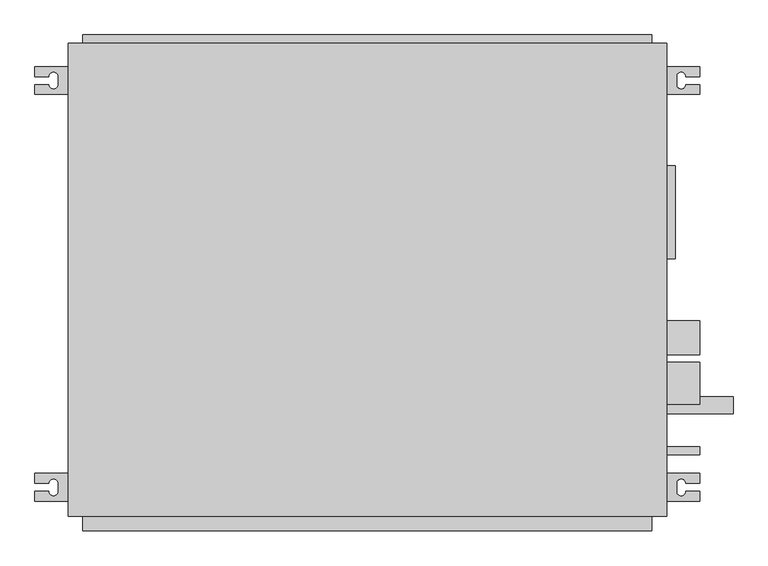
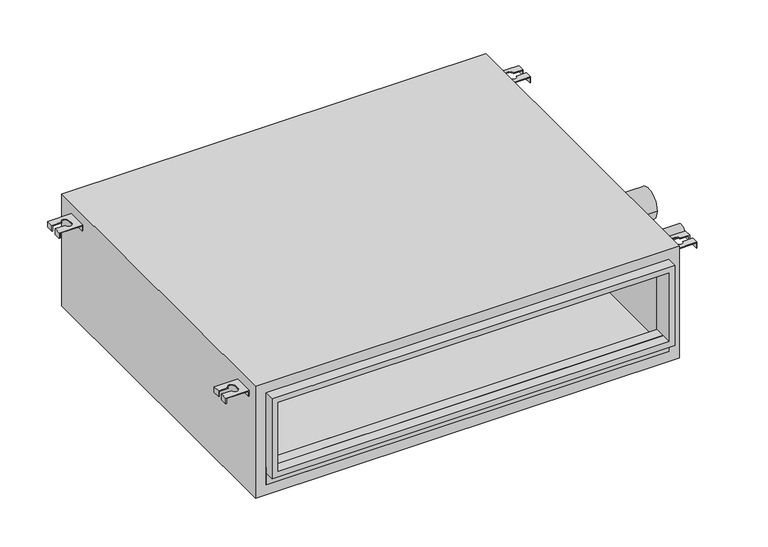
"""IFC4 building model written with IfcOpenShell, lengths in millimetres: proxy geometry, PEFY-P-NMAU-E_Medium_Static_Ducted : PEFY-P18NMAU-E."""

import ifcopenshell
import ifcopenshell.guid

model = None  # the IFC model being written
_history = None  # IfcOwnerHistory: only IFC2X3 demands one
_inside = {}  # id of a spatial element -> (the spatial element, [elements in it])
_under = {}  # id of a project, library or spatial element -> (it, [spatial elements below it])
_declared = {}  # id of a project -> (the project, [libraries it declares])
_typed = {}  # id of a type object -> (the type object, [elements of that type])
_made_of = {}  # id of a material, layer set ... -> (it, [elements and type objects made of it])


def new_model(schema):
    """Start an empty IFC model of exactly this schema.

    Asked for "IFC4X3", IfcOpenShell would pick the latest addendum, in which some entities
    have other attributes; the version numbers below select the first issue.
    IFC2X3 requires an IfcOwnerHistory on every rooted entity: one is made here for all.
    """
    global model, _history
    if schema == "IFC4X3":
        model = ifcopenshell.file(schema_version=(4, 3, 0, 0))
    else:
        model = ifcopenshell.file(schema=schema)
    _inside.clear()
    _under.clear()
    _declared.clear()
    _typed.clear()
    _made_of.clear()
    _history = None
    if model.schema == "IFC2X3":
        org = make("IfcOrganization", Name="unknown")
        user = make(
            "IfcPersonAndOrganization",
            ThePerson=make("IfcPerson", FamilyName="unknown"),
            TheOrganization=org,
        )
        app = make(
            "IfcApplication",
            ApplicationDeveloper=org,
            Version="unknown",
            ApplicationFullName="unknown",
            ApplicationIdentifier="unknown",
        )
        _history = make(
            "IfcOwnerHistory",
            OwningUser=user,
            OwningApplication=app,
            ChangeAction="ADDED",
            CreationDate=0,
        )
    return model


def make(cls, **values):
    """One entity of the class cls with the attributes given. An attribute that is None is left unset."""
    return model.create_entity(
        cls, **{name: value for name, value in values.items() if value is not None}
    )


def rooted(cls, **values):
    """An entity with a GlobalId (a new one), such as an element, a storey or a relation."""
    return make(cls, GlobalId=ifcopenshell.guid.new(), OwnerHistory=_history, **values)


def si_unit(unit_type, name, prefix=None):
    """IfcSIUnit, for example si_unit("LENGTHUNIT", "METRE", prefix="MILLI")."""
    return make("IfcSIUnit", UnitType=unit_type, Prefix=prefix, Name=name)


def assignment(units):
    """IfcUnitAssignment: the units of a project."""
    return None if units is None else make("IfcUnitAssignment", Units=units)


def point(xyz):
    """IfcCartesianPoint."""
    return None if xyz is None else make("IfcCartesianPoint", Coordinates=xyz)


def direction(xyz):
    """IfcDirection."""
    return None if xyz is None else make("IfcDirection", DirectionRatios=xyz)


def frame(location, z_axis=None, x_axis=None):
    """IfcAxis2Placement3D, a coordinate frame: its origin and axes. An axis left out is left unset."""
    return make(
        "IfcAxis2Placement3D",
        Location=point(location),
        Axis=direction(z_axis),
        RefDirection=direction(x_axis),
    )


def frame_2d(location, x_axis=None):
    """IfcAxis2Placement2D, a coordinate frame in the plane: its origin and x axis."""
    return make(
        "IfcAxis2Placement2D", Location=point(location), RefDirection=direction(x_axis)
    )


def origin():
    """The frame at (0, 0, 0) with its axes left unset."""
    return frame((0.0, 0.0, 0.0))


def place(relative_to, where):
    """IfcLocalPlacement: puts the frame where relative to a parent placement (None: the world)."""
    return make(
        "IfcLocalPlacement", PlacementRelTo=relative_to, RelativePlacement=where
    )


def context(
    kind, dimensions, precision=None, world=None, true_north=None, identifier=None
):
    """IfcGeometricRepresentationContext, for example the 3D "Model" context."""
    return make(
        "IfcGeometricRepresentationContext",
        ContextIdentifier=identifier,
        ContextType=kind,
        CoordinateSpaceDimension=dimensions,
        Precision=precision,
        WorldCoordinateSystem=world,
        TrueNorth=true_north,
    )


def project(units=None, contexts=None):
    """IfcProject with its units and contexts."""
    return rooted(
        "IfcProject",
        Name="project",
        RepresentationContexts=contexts,
        UnitsInContext=assignment(units),
    )


def spatial(cls, under=None, at=None, **own):
    """A site, building, storey or space (cls), placed at a placement, below another one or the project."""
    s = rooted(cls, ObjectPlacement=at, **own)
    if under is not None:
        _under.setdefault(under.id(), (under, []))[1].append(s)
    return s


def polyline(points):
    """IfcPolyline through the points."""
    return make("IfcPolyline", Points=[point(p) for p in points])


def circle_curve(where, radius):
    """IfcCircle in the frame where."""
    return make("IfcCircle", Position=where, Radius=radius)


def trimmed(basis, trim1, trim2, sense, master):
    """IfcTrimmedCurve: the piece of a basis curve between two trims."""
    return make(
        "IfcTrimmedCurve",
        BasisCurve=basis,
        Trim1=trim1,
        Trim2=trim2,
        SenseAgreement=sense,
        MasterRepresentation=master,
    )


def segment(curve, same_sense, transition):
    """IfcCompositeCurveSegment."""
    return make(
        "IfcCompositeCurveSegment",
        Transition=transition,
        SameSense=same_sense,
        ParentCurve=curve,
    )


def composite_curve(segments, self_intersect=None):
    """IfcCompositeCurve: segments joined end to end."""
    return make("IfcCompositeCurve", Segments=segments, SelfIntersect=self_intersect)


def outline(outer, holes=None, kind="AREA"):
    """IfcArbitraryClosedProfileDef: a profile drawn as a closed curve; with holes, ...WithVoids."""
    if holes is None:
        return make("IfcArbitraryClosedProfileDef", ProfileType=kind, OuterCurve=outer)
    return make(
        "IfcArbitraryProfileDefWithVoids",
        ProfileType=kind,
        OuterCurve=outer,
        InnerCurves=holes,
    )


def extrude(swept, where, along, depth):
    """IfcExtrudedAreaSolid: the profile swept, set in the frame where, extruded along a direction by depth."""
    return make(
        "IfcExtrudedAreaSolid",
        SweptArea=swept,
        Position=where,
        ExtrudedDirection=direction(along),
        Depth=depth,
    )


def shape(context_of_items, identifier, shape_type, items):
    """IfcShapeRepresentation: the items that make up one representation, for example the "Body"."""
    return make(
        "IfcShapeRepresentation",
        ContextOfItems=context_of_items,
        RepresentationIdentifier=identifier,
        RepresentationType=shape_type,
        Items=items,
    )


def source(mapping_origin, context_of_items, identifier, shape_type, items):
    """IfcRepresentationMap: a shape defined once, which mapped items show again and again."""
    return make(
        "IfcRepresentationMap",
        MappingOrigin=mapping_origin,
        MappedRepresentation=shape(context_of_items, identifier, shape_type, items),
    )


def transform(
    local_origin,
    x_axis=None,
    y_axis=None,
    z_axis=None,
    scale=None,
    scale2=None,
    scale3=None,
    uniform=True,
):
    """IfcCartesianTransformationOperator3D, or its non-uniform kind. x_axis, y_axis, z_axis: its Axis1, 2, 3."""
    if uniform:
        return make(
            "IfcCartesianTransformationOperator3D",
            Axis1=direction(x_axis),
            Axis2=direction(y_axis),
            LocalOrigin=point(local_origin),
            Scale=scale,
            Axis3=direction(z_axis),
        )
    return make(
        "IfcCartesianTransformationOperator3DnonUniform",
        Axis1=direction(x_axis),
        Axis2=direction(y_axis),
        LocalOrigin=point(local_origin),
        Scale=scale,
        Axis3=direction(z_axis),
        Scale2=scale2,
        Scale3=scale3,
    )


def mapped(mapping_source, mapping_target):
    """IfcMappedItem: shows the shape of a source again, moved by a transform."""
    return make(
        "IfcMappedItem", MappingSource=mapping_source, MappingTarget=mapping_target
    )


def made_of(thing, what):
    """Note that an element or type object is made of a material, layer set ...; save() writes the relation."""
    if what is not None:
        _made_of.setdefault(what.id(), (what, []))[1].append(thing)
    return thing


def element(
    cls,
    number,
    at=None,
    inside=None,
    cuts=None,
    type_object=None,
    material=None,
    context=None,
    identifier="Body",
    shape_type=None,
    held_by="IfcProductDefinitionShape",
    body=None,
    shapes=None,
    **own,
):
    """One element of the class cls, such as IfcWall. Its Tag is "e" and its number.

    at: its placement. inside: the storey or other place that contains it. cuts: it is an
    opening in that element (IfcRelVoidsElement). A single representation is given by context,
    identifier, shape_type and body (its items); several are given by shapes. held_by: the class
    of the entity that holds the representations. save() writes the other relations.
    """
    e = rooted(cls, Tag="e%d" % number, ObjectPlacement=at, **own)
    if body is not None:
        shapes = [shape(context, identifier, shape_type, body)]
    if shapes is not None:
        e.Representation = make(held_by, Representations=shapes)
    if inside is not None:
        _inside.setdefault(inside.id(), (inside, []))[1].append(e)
    if cuts is not None:
        rooted(
            "IfcRelVoidsElement", RelatingBuildingElement=cuts, RelatedOpeningElement=e
        )
    if type_object is not None:
        _typed.setdefault(type_object.id(), (type_object, []))[1].append(e)
    return made_of(e, material)


def aggregate(whole, parts):
    """IfcRelAggregates: a whole, such as a stair, and the parts it consists of."""
    return rooted("IfcRelAggregates", RelatingObject=whole, RelatedObjects=parts)


def save(model, path):
    """Write the relations noted so far, then the file.

    IfcRelAggregates (storeys below a building ...), IfcRelContainedInSpatialStructure (elements
    in a storey), IfcRelDefinesByType, IfcRelAssociatesMaterial and IfcRelDeclares: one each for
    every whole, place, type object, material and project.
    """
    for whole, parts in _under.values():
        aggregate(whole, parts)
    for where, things in _inside.values():
        rooted(
            "IfcRelContainedInSpatialStructure",
            RelatedElements=things,
            RelatingStructure=where,
        )
    for kind, things in _typed.values():
        rooted("IfcRelDefinesByType", RelatedObjects=things, RelatingType=kind)
    for what, things in _made_of.values():
        rooted("IfcRelAssociatesMaterial", RelatedObjects=things, RelatingMaterial=what)
    for by, libraries in _declared.values():
        rooted("IfcRelDeclares", RelatingContext=by, RelatedDefinitions=libraries)
    model.write(path)


def plane_surface(at):
    """IfcPlane: the flat surface through the origin of the frame at, square to its z axis."""
    return make("IfcPlane", Position=at)


def revolved_surface(curve, axis_point, axis_direction):
    """IfcSurfaceOfRevolution: the curve turned about the line through axis_point along axis_direction."""
    return make(
        "IfcSurfaceOfRevolution",
        SweptCurve=make("IfcArbitraryOpenProfileDef", ProfileType="CURVE", Curve=curve),
        AxisPosition=make("IfcAxis1Placement", Location=point(axis_point), Axis=direction(axis_direction)),
    )


def advanced_brep(points, edges, surfaces, faces):
    """IfcAdvancedBrep: a solid bounded by faces that lie on surfaces and meet in shared edges.

    An edge is (start, end): straight between two places in points (the first is 0);
    or (start, end, curve); or (start, end, curve, False) where it runs against its curve.
    A face is (place in surfaces, loops), or (place, loops, False) where it looks against
    its surface's normal. A loop lists edges by number (the first is 1), with a minus sign
    where the edge is run from its end to its start. The first loop is the outer one.
    """
    corners = [point(p) for p in points]
    vertices = [make("IfcVertexPoint", VertexGeometry=c) for c in corners]
    made = []
    for start, end, *more in edges:
        made.append(
            make(
                "IfcEdgeCurve",
                EdgeStart=vertices[start],
                EdgeEnd=vertices[end],
                EdgeGeometry=more[0] if more else make("IfcPolyline", Points=[corners[start], corners[end]]),
                SameSense=more[1] if len(more) > 1 else True,
            )
        )
    hull = []
    for where, loops, *sense in faces:
        bounds = []
        for j, loop in enumerate(loops):
            ring = [make("IfcOrientedEdge", EdgeElement=made[abs(k) - 1], Orientation=k > 0) for k in loop]
            bounds.append(
                make(
                    "IfcFaceOuterBound" if j == 0 else "IfcFaceBound",
                    Bound=make("IfcEdgeLoop", EdgeList=ring),
                    Orientation=True,
                )
            )
        hull.append(make("IfcAdvancedFace", Bounds=bounds, FaceSurface=surfaces[where], SameSense=sense[0] if sense else True))
    return make("IfcAdvancedBrep", Outer=make("IfcClosedShell", CfsFaces=hull))


def mechanical_equipment_7e022f85(model_context):
    return source(origin(), model_context, "Body", "SolidModel", [
        advanced_brep(
        [(-510.074743, -231.05, 249.2375), (-510.074743, -246.05, 249.2375), (-489.068493, -246.05, 249.2375), (-475.068493, -246.05, 249.2375), (-475.068493, -258.05, 249.2375), (-489.068493, -258.05, 249.2375), (-510.074743, -258.05, 249.2375), (-510.074743, -273.05, 249.2375), (-460.068493, -273.05, 249.2375), (-460.068493, -231.05, 249.2375), (-510.074743, -231.05, 236.4972162), (-508.486743, -231.05, 236.4972162), (-508.486743, -246.05, 236.4972162), (-510.074743, -246.05, 236.4972162), (-508.486743, -273.05, 236.4972162), (-510.074743, -273.05, 236.4972162), (-510.074743, -258.05, 236.4972162), (-508.486743, -258.05, 236.4972162), (-460.068493, -231.05, 236.4972162), (-460.068493, -273.05, 236.4972162), (-461.656493, -273.05, 236.4972162), (-461.656493, -231.05, 236.4972162), (-508.486743, -246.05, 247.65), (-489.068493, -246.05, 247.65), (-508.486743, -231.05, 247.65), (-461.656493, -231.05, 247.65), (-508.486743, -258.05, 247.65), (-508.486743, -273.05, 247.65), (-489.068493, -258.05, 247.65), (-461.656493, -273.05, 247.65), (-475.068493, -258.05, 247.65), (-475.068493, -246.05, 247.65)],
        [
            (0, 1),
            (1, 2),
            (2, 3, circle_curve(frame((-482.068493, -246.05, 249.2375), z_axis=(0.0, 0.0, -1.0), x_axis=(1.0, 0.0, 0.0)), 7.0)),
            (3, 4),
            (4, 5, circle_curve(frame((-482.068493, -258.05, 249.2375), z_axis=(0.0, 0.0, -1.0), x_axis=(1.0, 0.0, 0.0)), 7.0)),
            (5, 6),
            (6, 7),
            (7, 8),
            (8, 9),
            (9, 0),
            (10, 11),
            (11, 12),
            (12, 13),
            (13, 10),
            (14, 15),
            (15, 16),
            (16, 17),
            (17, 14),
            (18, 19),
            (19, 20),
            (20, 21),
            (21, 18),
            (13, 1),
            (0, 10),
            (12, 22),
            (22, 23),
            (23, 2),
            (11, 24),
            (24, 22),
            (9, 18),
            (21, 25),
            (25, 24),
            (17, 26),
            (26, 27),
            (27, 14),
            (5, 28),
            (28, 26),
            (16, 6),
            (15, 7),
            (27, 29),
            (29, 20),
            (19, 8),
            (29, 25),
            (30, 31),
            (31, 23, circle_curve(frame((-482.068493, -246.05, 247.65), z_axis=(0.0, 0.0, 1.0), x_axis=(1.0, 0.0, 0.0)), 7.0)),
            (28, 30, circle_curve(frame((-482.068493, -258.05, 247.65), z_axis=(0.0, 0.0, 1.0), x_axis=(1.0, 0.0, 0.0)), 7.0)),
            (4, 30),
            (31, 3),
        ],
        [
            plane_surface(frame((-510.074743, -231.05, 249.2375), z_axis=(0.0, 0.0, 1.0), x_axis=(0.0, -1.0, 0.0))),
            plane_surface(frame((-510.074743, -231.05, 236.4972162), z_axis=(0.0, 0.0, -1.0), x_axis=(0.0, 1.0, 0.0))),
            plane_surface(frame((-510.074743, -231.05, 249.2375), z_axis=(-1.0, 0.0, 0.0), x_axis=(0.0, 0.0, -1.0))),
            plane_surface(frame((-510.074743, -246.05, 249.2375), z_axis=(0.0, -1.0, 0.0), x_axis=(0.0, 0.0, -1.0))),
            plane_surface(frame((-508.486743, -246.05, 249.2375), z_axis=(1.0, 0.0, 0.0), x_axis=(0.0, 0.0, -1.0))),
            plane_surface(frame((-508.486743, -231.05, 249.2375), z_axis=(0.0, 1.0, 0.0), x_axis=(0.0, 0.0, -1.0))),
            plane_surface(frame((-508.486743, -273.05, 249.2375), z_axis=(1.0, 0.0, 0.0), x_axis=(0.0, 0.0, -1.0))),
            plane_surface(frame((-508.486743, -258.05, 249.2375), z_axis=(0.0, 1.0, 0.0), x_axis=(0.0, 0.0, -1.0))),
            plane_surface(frame((-510.074743, -258.05, 249.2375), z_axis=(-1.0, 0.0, 0.0), x_axis=(0.0, 0.0, -1.0))),
            plane_surface(frame((-510.074743, -273.05, 249.2375), z_axis=(0.0, -1.0, 0.0), x_axis=(0.0, 0.0, -1.0))),
            plane_surface(frame((-461.656493, -231.05, 249.2375), z_axis=(-1.0, 0.0, 0.0), x_axis=(0.0, 0.0, -1.0))),
            plane_surface(frame((-460.068493, -273.05, 249.2375), z_axis=(1.0, 0.0, 0.0), x_axis=(0.0, 0.0, -1.0))),
            plane_surface(frame((-475.068493, -258.05, 247.65), z_axis=(0.0, 0.0, -1.0), x_axis=(0.0, 1.0, 0.0))),
            revolved_surface(polyline([(-475.068493, -258.05, 247.65), (-475.068493, -258.05, 249.2375)]), (-482.068493, -258.05, 247.65), (0.0, 0.0, -1.0)),
            revolved_surface(polyline([(-475.068493, -246.05, 247.65), (-475.068493, -246.05, 249.2375)]), (-482.068493, -246.05, 247.65), (0.0, 0.0, -1.0)),
            plane_surface(frame((-475.068493, -246.05, 249.2375), z_axis=(-1.0, 0.0, 0.0), x_axis=(0.0, 0.0, -1.0))),
        ],
        [
            (0, [[1, 2, 3, 4, 5, 6, 7, 8, 9, 10]]),
            (1, [[11, 12, 13, 14]]),
            (1, [[15, 16, 17, 18]]),
            (1, [[19, 20, 21, 22]]),
            (2, [[23, -1, 24, -14]]),
            (3, [[-2, -23, -13, 25, 26, 27]]),
            (4, [[-12, 28, 29, -25]]),
            (5, [[-10, 30, -22, 31, 32, -28, -11, -24]]),
            (6, [[-18, 33, 34, 35]]),
            (7, [[-6, 36, 37, -33, -17, 38]]),
            (8, [[39, -7, -38, -16]]),
            (9, [[-8, -39, -15, -35, 40, 41, -20, 42]]),
            (10, [[-21, -41, 43, -31]]),
            (11, [[-30, -9, -42, -19]]),
            (12, [[44, 45, -26, -29, -32, -43, -40, -34, -37, 46]]),
            (13, [[-5, 47, -46, -36]]),
            (14, [[-3, -27, -45, 48]]),
            (15, [[-4, -48, -44, -47]]),
        ],
    ),
        advanced_brep(
        [(490.050257, -231.05, 249.2375), (440.044007, -231.05, 249.2375), (440.044007, -273.05, 249.2375), (490.050257, -273.05, 249.2375), (490.050257, -258.05, 249.2375), (469.044007, -258.05, 249.2375), (455.044007, -258.05, 249.2375), (455.044007, -246.05, 249.2375), (469.044007, -246.05, 249.2375), (490.050257, -246.05, 249.2375), (490.050257, -231.05, 236.4972162), (490.050257, -246.05, 236.4972162), (488.462257, -246.05, 236.4972162), (488.462257, -231.05, 236.4972162), (488.462257, -273.05, 236.4972162), (488.462257, -258.05, 236.4972162), (490.050257, -258.05, 236.4972162), (490.050257, -273.05, 236.4972162), (440.044007, -231.05, 236.4972162), (441.632007, -231.05, 236.4972162), (441.632007, -273.05, 236.4972162), (440.044007, -273.05, 236.4972162), (469.044007, -246.05, 247.65), (488.462257, -246.05, 247.65), (488.462257, -231.05, 247.65), (441.632007, -231.05, 247.65), (488.462257, -273.05, 247.65), (488.462257, -258.05, 247.65), (469.044007, -258.05, 247.65), (441.632007, -273.05, 247.65), (455.044007, -258.05, 247.65), (455.044007, -246.05, 247.65)],
        [
            (0, 1),
            (1, 2),
            (2, 3),
            (3, 4),
            (4, 5),
            (5, 6, circle_curve(frame((462.044007, -258.05, 249.2375), z_axis=(0.0, 0.0, -1.0), x_axis=(-1.0, 0.0, 0.0)), 7.0)),
            (6, 7),
            (7, 8, circle_curve(frame((462.044007, -246.05, 249.2375), z_axis=(0.0, 0.0, -1.0), x_axis=(-1.0, 0.0, 0.0)), 7.0)),
            (8, 9),
            (9, 0),
            (10, 11),
            (11, 12),
            (12, 13),
            (13, 10),
            (14, 15),
            (15, 16),
            (16, 17),
            (17, 14),
            (18, 19),
            (19, 20),
            (20, 21),
            (21, 18),
            (10, 0),
            (9, 11),
            (8, 22),
            (22, 23),
            (23, 12),
            (23, 24),
            (24, 13),
            (24, 25),
            (25, 19),
            (18, 1),
            (14, 26),
            (26, 27),
            (27, 15),
            (4, 16),
            (27, 28),
            (28, 5),
            (3, 17),
            (2, 21),
            (20, 29),
            (29, 26),
            (25, 29),
            (30, 28, circle_curve(frame((462.044007, -258.05, 247.65), z_axis=(0.0, 0.0, 1.0), x_axis=(-1.0, 0.0, 0.0)), 7.0)),
            (22, 31, circle_curve(frame((462.044007, -246.05, 247.65), z_axis=(0.0, 0.0, 1.0), x_axis=(-1.0, 0.0, 0.0)), 7.0)),
            (31, 30),
            (30, 6),
            (7, 31),
        ],
        [
            plane_surface(frame((490.050257, -231.05, 249.2375), z_axis=(0.0, 0.0, 1.0), x_axis=(0.0, -1.0, 0.0))),
            plane_surface(frame((490.050257, -231.05, 236.4972162), z_axis=(0.0, 0.0, -1.0), x_axis=(0.0, 1.0, 0.0))),
            plane_surface(frame((490.050257, -231.05, 249.2375), z_axis=(1.0, 0.0, 0.0), x_axis=(0.0, 0.0, -1.0))),
            plane_surface(frame((490.050257, -246.05, 249.2375), z_axis=(0.0, -1.0, 0.0), x_axis=(0.0, 0.0, -1.0))),
            plane_surface(frame((488.462257, -246.05, 249.2375), z_axis=(-1.0, 0.0, 0.0), x_axis=(0.0, 0.0, -1.0))),
            plane_surface(frame((488.462257, -231.05, 249.2375), z_axis=(0.0, 1.0, 0.0), x_axis=(0.0, 0.0, -1.0))),
            plane_surface(frame((488.462257, -273.05, 249.2375), z_axis=(-1.0, 0.0, 0.0), x_axis=(0.0, 0.0, -1.0))),
            plane_surface(frame((488.462257, -258.05, 249.2375), z_axis=(0.0, 1.0, 0.0), x_axis=(0.0, 0.0, -1.0))),
            plane_surface(frame((490.050257, -258.05, 249.2375), z_axis=(1.0, 0.0, 0.0), x_axis=(0.0, 0.0, -1.0))),
            plane_surface(frame((490.050257, -273.05, 249.2375), z_axis=(0.0, -1.0, 0.0), x_axis=(0.0, 0.0, -1.0))),
            plane_surface(frame((441.632007, -231.05, 249.2375), z_axis=(1.0, 0.0, 0.0), x_axis=(0.0, 0.0, -1.0))),
            plane_surface(frame((440.044007, -273.05, 249.2375), z_axis=(-1.0, 0.0, 0.0), x_axis=(0.0, 0.0, -1.0))),
            plane_surface(frame((455.044007, -258.05, 247.65), z_axis=(0.0, 0.0, -1.0), x_axis=(0.0, 1.0, 0.0))),
            revolved_surface(polyline([(455.044007, -258.05, 247.65), (455.044007, -258.05, 249.2375)]), (462.044007, -258.05, 247.65), (0.0, 0.0, -1.0)),
            revolved_surface(polyline([(455.044007, -246.05, 247.65), (455.044007, -246.05, 249.2375)]), (462.044007, -246.05, 247.65), (0.0, 0.0, -1.0)),
            plane_surface(frame((455.044007, -246.05, 249.2375), z_axis=(1.0, 0.0, 0.0), x_axis=(0.0, 0.0, -1.0))),
        ],
        [
            (0, [[1, 2, 3, 4, 5, 6, 7, 8, 9, 10]]),
            (1, [[11, 12, 13, 14]]),
            (1, [[15, 16, 17, 18]]),
            (1, [[19, 20, 21, 22]]),
            (2, [[-11, 23, -10, 24]]),
            (3, [[25, 26, 27, -12, -24, -9]]),
            (4, [[-27, 28, 29, -13]]),
            (5, [[-23, -14, -29, 30, 31, -19, 32, -1]]),
            (6, [[33, 34, 35, -15]]),
            (7, [[36, -16, -35, 37, 38, -5]]),
            (8, [[-17, -36, -4, 39]]),
            (9, [[40, -21, 41, 42, -33, -18, -39, -3]]),
            (10, [[-31, 43, -41, -20]]),
            (11, [[-22, -40, -2, -32]]),
            (12, [[44, -37, -34, -42, -43, -30, -28, -26, 45, 46]]),
            (13, [[-38, -44, 47, -6]]),
            (14, [[48, -45, -25, -8]]),
            (15, [[-47, -46, -48, -7]]),
        ],
    ),
        advanced_brep(
        [(-510.074743, 339.0, 249.2375), (-460.068493, 339.0, 249.2375), (-460.068493, 381.0, 249.2375), (-510.074743, 381.0, 249.2375), (-510.074743, 366.0, 249.2375), (-489.068493, 366.0, 249.2375), (-475.068493, 366.0, 249.2375), (-475.068493, 354.0, 249.2375), (-489.068493, 354.0, 249.2375), (-510.074743, 354.0, 249.2375), (-510.074743, 339.0, 236.4972162), (-510.074743, 354.0, 236.4972162), (-508.486743, 354.0, 236.4972162), (-508.486743, 339.0, 236.4972162), (-508.486743, 381.0, 236.4972162), (-508.486743, 366.0, 236.4972162), (-510.074743, 366.0, 236.4972162), (-510.074743, 381.0, 236.4972162), (-460.068493, 339.0, 236.4972162), (-461.656493, 339.0, 236.4972162), (-461.656493, 381.0, 236.4972162), (-460.068493, 381.0, 236.4972162), (-489.068493, 354.0, 247.65), (-508.486743, 354.0, 247.65), (-508.486743, 339.0, 247.65), (-461.656493, 339.0, 247.65), (-508.486743, 381.0, 247.65), (-508.486743, 366.0, 247.65), (-489.068493, 366.0, 247.65), (-461.656493, 381.0, 247.65), (-475.068493, 366.0, 247.65), (-475.068493, 354.0, 247.65)],
        [
            (0, 1),
            (1, 2),
            (2, 3),
            (3, 4),
            (4, 5),
            (5, 6, circle_curve(frame((-482.068493, 366.0, 249.2375), z_axis=(0.0, 0.0, -1.0), x_axis=(1.0, 0.0, 0.0)), 7.0)),
            (6, 7),
            (7, 8, circle_curve(frame((-482.068493, 354.0, 249.2375), z_axis=(0.0, 0.0, -1.0), x_axis=(1.0, 0.0, 0.0)), 7.0)),
            (8, 9),
            (9, 0),
            (10, 11),
            (11, 12),
            (12, 13),
            (13, 10),
            (14, 15),
            (15, 16),
            (16, 17),
            (17, 14),
            (18, 19),
            (19, 20),
            (20, 21),
            (21, 18),
            (10, 0),
            (9, 11),
            (8, 22),
            (22, 23),
            (23, 12),
            (23, 24),
            (24, 13),
            (24, 25),
            (25, 19),
            (18, 1),
            (14, 26),
            (26, 27),
            (27, 15),
            (4, 16),
            (27, 28),
            (28, 5),
            (3, 17),
            (2, 21),
            (20, 29),
            (29, 26),
            (25, 29),
            (30, 28, circle_curve(frame((-482.068493, 366.0, 247.65), z_axis=(0.0, 0.0, 1.0), x_axis=(1.0, 0.0, 0.0)), 7.0)),
            (22, 31, circle_curve(frame((-482.068493, 354.0, 247.65), z_axis=(0.0, 0.0, 1.0), x_axis=(1.0, 0.0, 0.0)), 7.0)),
            (31, 30),
            (30, 6),
            (7, 31),
        ],
        [
            plane_surface(frame((-510.074743, 339.0, 249.2375), z_axis=(0.0, 0.0, 1.0), x_axis=(0.0, 1.0, 0.0))),
            plane_surface(frame((-510.074743, 339.0, 236.4972162), z_axis=(0.0, 0.0, -1.0), x_axis=(0.0, -1.0, 0.0))),
            plane_surface(frame((-510.074743, 339.0, 249.2375), z_axis=(-1.0, 0.0, 0.0), x_axis=(0.0, 0.0, -1.0))),
            plane_surface(frame((-510.074743, 354.0, 249.2375), z_axis=(0.0, 1.0, 0.0), x_axis=(0.0, 0.0, -1.0))),
            plane_surface(frame((-508.486743, 354.0, 249.2375), z_axis=(1.0, 0.0, 0.0), x_axis=(0.0, 0.0, -1.0))),
            plane_surface(frame((-508.486743, 339.0, 249.2375), z_axis=(0.0, -1.0, 0.0), x_axis=(0.0, 0.0, -1.0))),
            plane_surface(frame((-508.486743, 381.0, 249.2375), z_axis=(1.0, 0.0, 0.0), x_axis=(0.0, 0.0, -1.0))),
            plane_surface(frame((-508.486743, 366.0, 249.2375), z_axis=(0.0, -1.0, 0.0), x_axis=(0.0, 0.0, -1.0))),
            plane_surface(frame((-510.074743, 366.0, 249.2375), z_axis=(-1.0, 0.0, 0.0), x_axis=(0.0, 0.0, -1.0))),
            plane_surface(frame((-510.074743, 381.0, 249.2375), z_axis=(0.0, 1.0, 0.0), x_axis=(0.0, 0.0, -1.0))),
            plane_surface(frame((-461.656493, 339.0, 249.2375), z_axis=(-1.0, 0.0, 0.0), x_axis=(0.0, 0.0, -1.0))),
            plane_surface(frame((-460.068493, 381.0, 249.2375), z_axis=(1.0, 0.0, 0.0), x_axis=(0.0, 0.0, -1.0))),
            plane_surface(frame((-475.068493, 366.0, 247.65), z_axis=(0.0, 0.0, -1.0), x_axis=(0.0, -1.0, 0.0))),
            revolved_surface(polyline([(-475.068493, 366.0, 247.65), (-475.068493, 366.0, 249.2375)]), (-482.068493, 366.0, 247.65), (0.0, 0.0, -1.0)),
            revolved_surface(polyline([(-475.068493, 354.0, 247.65), (-475.068493, 354.0, 249.2375)]), (-482.068493, 354.0, 247.65), (0.0, 0.0, -1.0)),
            plane_surface(frame((-475.068493, 354.0, 249.2375), z_axis=(-1.0, 0.0, 0.0), x_axis=(0.0, 0.0, -1.0))),
        ],
        [
            (0, [[1, 2, 3, 4, 5, 6, 7, 8, 9, 10]]),
            (1, [[11, 12, 13, 14]]),
            (1, [[15, 16, 17, 18]]),
            (1, [[19, 20, 21, 22]]),
            (2, [[-11, 23, -10, 24]]),
            (3, [[25, 26, 27, -12, -24, -9]]),
            (4, [[-27, 28, 29, -13]]),
            (5, [[-23, -14, -29, 30, 31, -19, 32, -1]]),
            (6, [[33, 34, 35, -15]]),
            (7, [[36, -16, -35, 37, 38, -5]]),
            (8, [[-17, -36, -4, 39]]),
            (9, [[40, -21, 41, 42, -33, -18, -39, -3]]),
            (10, [[-31, 43, -41, -20]]),
            (11, [[-22, -40, -2, -32]]),
            (12, [[44, -37, -34, -42, -43, -30, -28, -26, 45, 46]]),
            (13, [[-38, -44, 47, -6]]),
            (14, [[48, -45, -25, -8]]),
            (15, [[-47, -46, -48, -7]]),
        ],
    ),
        advanced_brep(
        [(490.050257, 339.0, 249.2375), (490.050257, 354.0, 249.2375), (469.044007, 354.0, 249.2375), (455.044007, 354.0, 249.2375), (455.044007, 366.0, 249.2375), (469.044007, 366.0, 249.2375), (490.050257, 366.0, 249.2375), (490.050257, 381.0, 249.2375), (440.044007, 381.0, 249.2375), (440.044007, 339.0, 249.2375), (490.050257, 339.0, 236.4972162), (488.462257, 339.0, 236.4972162), (488.462257, 354.0, 236.4972162), (490.050257, 354.0, 236.4972162), (488.462257, 381.0, 236.4972162), (490.050257, 381.0, 236.4972162), (490.050257, 366.0, 236.4972162), (488.462257, 366.0, 236.4972162), (440.044007, 339.0, 236.4972162), (440.044007, 381.0, 236.4972162), (441.632007, 381.0, 236.4972162), (441.632007, 339.0, 236.4972162), (488.462257, 354.0, 247.65), (469.044007, 354.0, 247.65), (488.462257, 339.0, 247.65), (441.632007, 339.0, 247.65), (488.462257, 366.0, 247.65), (488.462257, 381.0, 247.65), (469.044007, 366.0, 247.65), (441.632007, 381.0, 247.65), (455.044007, 366.0, 247.65), (455.044007, 354.0, 247.65)],
        [
            (0, 1),
            (1, 2),
            (2, 3, circle_curve(frame((462.044007, 354.0, 249.2375), z_axis=(0.0, 0.0, -1.0), x_axis=(-1.0, 0.0, 0.0)), 7.0)),
            (3, 4),
            (4, 5, circle_curve(frame((462.044007, 366.0, 249.2375), z_axis=(0.0, 0.0, -1.0), x_axis=(-1.0, 0.0, 0.0)), 7.0)),
            (5, 6),
            (6, 7),
            (7, 8),
            (8, 9),
            (9, 0),
            (10, 11),
            (11, 12),
            (12, 13),
            (13, 10),
            (14, 15),
            (15, 16),
            (16, 17),
            (17, 14),
            (18, 19),
            (19, 20),
            (20, 21),
            (21, 18),
            (13, 1),
            (0, 10),
            (12, 22),
            (22, 23),
            (23, 2),
            (11, 24),
            (24, 22),
            (9, 18),
            (21, 25),
            (25, 24),
            (17, 26),
            (26, 27),
            (27, 14),
            (5, 28),
            (28, 26),
            (16, 6),
            (15, 7),
            (27, 29),
            (29, 20),
            (19, 8),
            (29, 25),
            (30, 31),
            (31, 23, circle_curve(frame((462.044007, 354.0, 247.65), z_axis=(0.0, 0.0, 1.0), x_axis=(-1.0, 0.0, 0.0)), 7.0)),
            (28, 30, circle_curve(frame((462.044007, 366.0, 247.65), z_axis=(0.0, 0.0, 1.0), x_axis=(-1.0, 0.0, 0.0)), 7.0)),
            (4, 30),
            (31, 3),
        ],
        [
            plane_surface(frame((490.050257, 339.0, 249.2375), z_axis=(0.0, 0.0, 1.0), x_axis=(0.0, 1.0, 0.0))),
            plane_surface(frame((490.050257, 339.0, 236.4972162), z_axis=(0.0, 0.0, -1.0), x_axis=(0.0, -1.0, 0.0))),
            plane_surface(frame((490.050257, 339.0, 249.2375), z_axis=(1.0, 0.0, 0.0), x_axis=(0.0, 0.0, -1.0))),
            plane_surface(frame((490.050257, 354.0, 249.2375), z_axis=(0.0, 1.0, 0.0), x_axis=(0.0, 0.0, -1.0))),
            plane_surface(frame((488.462257, 354.0, 249.2375), z_axis=(-1.0, 0.0, 0.0), x_axis=(0.0, 0.0, -1.0))),
            plane_surface(frame((488.462257, 339.0, 249.2375), z_axis=(0.0, -1.0, 0.0), x_axis=(0.0, 0.0, -1.0))),
            plane_surface(frame((488.462257, 381.0, 249.2375), z_axis=(-1.0, 0.0, 0.0), x_axis=(0.0, 0.0, -1.0))),
            plane_surface(frame((488.462257, 366.0, 249.2375), z_axis=(0.0, -1.0, 0.0), x_axis=(0.0, 0.0, -1.0))),
            plane_surface(frame((490.050257, 366.0, 249.2375), z_axis=(1.0, 0.0, 0.0), x_axis=(0.0, 0.0, -1.0))),
            plane_surface(frame((490.050257, 381.0, 249.2375), z_axis=(0.0, 1.0, 0.0), x_axis=(0.0, 0.0, -1.0))),
            plane_surface(frame((441.632007, 339.0, 249.2375), z_axis=(1.0, 0.0, 0.0), x_axis=(0.0, 0.0, -1.0))),
            plane_surface(frame((440.044007, 381.0, 249.2375), z_axis=(-1.0, 0.0, 0.0), x_axis=(0.0, 0.0, -1.0))),
            plane_surface(frame((455.044007, 366.0, 247.65), z_axis=(0.0, 0.0, -1.0), x_axis=(0.0, -1.0, 0.0))),
            revolved_surface(polyline([(455.044007, 366.0, 247.65), (455.044007, 366.0, 249.2375)]), (462.044007, 366.0, 247.65), (0.0, 0.0, -1.0)),
            revolved_surface(polyline([(455.044007, 354.0, 247.65), (455.044007, 354.0, 249.2375)]), (462.044007, 354.0, 247.65), (0.0, 0.0, -1.0)),
            plane_surface(frame((455.044007, 354.0, 249.2375), z_axis=(1.0, 0.0, 0.0), x_axis=(0.0, 0.0, -1.0))),
        ],
        [
            (0, [[1, 2, 3, 4, 5, 6, 7, 8, 9, 10]]),
            (1, [[11, 12, 13, 14]]),
            (1, [[15, 16, 17, 18]]),
            (1, [[19, 20, 21, 22]]),
            (2, [[23, -1, 24, -14]]),
            (3, [[-2, -23, -13, 25, 26, 27]]),
            (4, [[-12, 28, 29, -25]]),
            (5, [[-10, 30, -22, 31, 32, -28, -11, -24]]),
            (6, [[-18, 33, 34, 35]]),
            (7, [[-6, 36, 37, -33, -17, 38]]),
            (8, [[39, -7, -38, -16]]),
            (9, [[-8, -39, -15, -35, 40, 41, -20, 42]]),
            (10, [[-21, -41, 43, -31]]),
            (11, [[-30, -9, -42, -19]]),
            (12, [[44, 45, -26, -29, -32, -43, -40, -34, -37, 46]]),
            (13, [[-5, 47, -46, -36]]),
            (14, [[-3, -27, -45, 48]]),
            (15, [[-4, -48, -44, -47]]),
        ],
    ),
        extrude(outline(polyline([(417.819007, -295.275), (-437.843493, -295.275), (-437.843493, -273.05), (417.819007, -273.05), (417.819007, -295.275)])), frame((0.0, 0.0, 42.8625), z_axis=(0.0, 0.0, 1.0), x_axis=(1.0, 0.0, 0.0)), (0.0, 0.0, 1.0), 39.6875),
        extrude(outline(polyline([(249.2375, 417.819007), (249.2375, -437.843493), (69.85, -437.843493), (69.85, 417.819007), (249.2375, 417.819007)]), holes=[polyline([(82.55, 405.119007), (82.55, -425.143493), (236.5375, -425.143493), (236.5375, 405.119007), (82.55, 405.119007)])]), frame((0.0, -317.5, 0.0), z_axis=(0.0, 1.0, 0.0), x_axis=(0.0, 0.0, 1.0)), (0.0, 0.0, 1.0), 44.45),
        extrude(outline(polyline([(417.819007, 415.925), (-437.843493, 415.925), (-437.843493, 428.625), (417.819007, 428.625), (417.819007, 415.925)])), frame((0.0, 0.0, 42.8625), z_axis=(0.0, 0.0, 1.0), x_axis=(1.0, 0.0, 0.0)), (0.0, 0.0, 1.0), 206.375),
        extrude(outline(polyline([(271.4625, 440.044007), (271.4625, -460.068493), (20.6375, -460.068493), (20.6375, 440.044007), (271.4625, 440.044007)]), holes=[polyline([(42.8625, -437.843493), (249.2375, -437.843493), (249.2375, 417.819007), (42.8625, 417.819007), (42.8625, -437.843493)])]), frame((0.0, -295.275, 0.0), z_axis=(0.0, 1.0, 0.0), x_axis=(0.0, 0.0, 1.0)), (0.0, 0.0, 1.0), 711.2),
        extrude(outline(composite_curve([segment(trimmed(circle_curve(frame_2d((-26.9875, 109.5375)), 25.4), [point((-1.5875, 109.5375))], [point((-52.3875, 109.5375))], False, "CARTESIAN"), True, "CONTINUOUS"), segment(trimmed(circle_curve(frame_2d((-26.9875, 109.5375)), 25.4), [point((-52.3875, 109.5375))], [point((-1.5875, 109.5375))], False, "CARTESIAN"), True, "CONTINUOUS")], self_intersect=False)), frame((440.044007, 0.0, 0.0), z_axis=(1.0, 0.0, 0.0), x_axis=(0.0, 1.0, 0.0)), (0.0, 0.0, 1.0), 50.00625),
        extrude(outline(composite_curve([segment(trimmed(circle_curve(frame_2d((-128.5875, 171.45)), 12.7), [point((-115.8875, 171.45))], [point((-141.2875, 171.45))], False, "CARTESIAN"), True, "CONTINUOUS"), segment(trimmed(circle_curve(frame_2d((-128.5875, 171.45)), 12.7), [point((-141.2875, 171.45))], [point((-115.8875, 171.45))], False, "CARTESIAN"), True, "CONTINUOUS")], self_intersect=False)), frame((440.044007, 0.0, 0.0), z_axis=(1.0, 0.0, 0.0), x_axis=(0.0, 1.0, 0.0)), (0.0, 0.0, 1.0), 100.0125),
        extrude(outline(composite_curve([segment(trimmed(circle_curve(frame_2d((-95.25, 230.1875)), 31.75), [point((-63.5, 230.1875))], [point((-127.0, 230.1875))], False, "CARTESIAN"), True, "CONTINUOUS"), segment(trimmed(circle_curve(frame_2d((-95.25, 230.1875)), 31.75), [point((-127.0, 230.1875))], [point((-63.5, 230.1875))], False, "CARTESIAN"), True, "CONTINUOUS")], self_intersect=False)), frame((440.044007, 0.0, 0.0), z_axis=(1.0, 0.0, 0.0), x_axis=(0.0, 1.0, 0.0)), (0.0, 0.0, 1.0), 50.00625),
        extrude(outline(composite_curve([segment(trimmed(circle_curve(frame_2d((-196.85, 104.775)), 6.35), [point((-190.5, 104.775))], [point((-203.2, 104.775))], False, "CARTESIAN"), True, "CONTINUOUS"), segment(trimmed(circle_curve(frame_2d((-196.85, 104.775)), 6.35), [point((-203.2, 104.775))], [point((-190.5, 104.775))], False, "CARTESIAN"), True, "CONTINUOUS")], self_intersect=False)), frame((440.044007, 0.0, 0.0), z_axis=(1.0, 0.0, 0.0), x_axis=(0.0, 1.0, 0.0)), (0.0, 0.0, 1.0), 50.00625),
        extrude(outline(polyline([(452.744007, 231.84375), (452.744007, 92.14375), (440.044007, 92.14375), (440.044007, 231.84375), (452.744007, 231.84375)])), frame((0.0, 0.0, 42.8625), z_axis=(0.0, 0.0, 1.0), x_axis=(1.0, 0.0, 0.0)), (0.0, 0.0, 1.0), 187.325),
    ])


if __name__ == "__main__":
    model = new_model("IFC4")
    model_context = context("Model", 3, world=origin())
    ifc_project = project(units=[si_unit("LENGTHUNIT", "METRE", prefix="MILLI")], contexts=[model_context])
    site = spatial("IfcSite", under=ifc_project)
    building = spatial("IfcBuilding", under=site)
    placement = place(None, origin())
    mechanical_equipment_shape = mechanical_equipment_7e022f85(model_context)
    element("IfcBuildingElementProxy", 1, Name="PEFY-P-NMAU-E_Medium_Static_Ducted : PEFY-P18NMAU-E", ObjectType="PEFY-P-NMAU-E_Medium_Static_Ducted : PEFY-P18NMAU-E", at=placement, inside=building, context=model_context, shape_type="MappedRepresentation", body=[
        mapped(mechanical_equipment_shape, transform((0.0, 0.0, 0.0), x_axis=(1.0, 0.0, 0.0), y_axis=(0.0, 1.0, 0.0), z_axis=(0.0, 0.0, 1.0))),
    ])
    save(model, "model.ifc")

# Revit data of these elements
# Type "PEFY-P-NMAU-E_Medium_Static_Ducted : PEFY-P18NMAU-E"
#   Wiring (Min.size of wire) = "1/8"
#   Wiring (Amperage of wire breaker) = "15 A"
#   Voltage Options = "208/230 VAC"
#   Unit Weight (LBS) = "58"
#   Temperature set range Remote controller Heating = "63 to 83 F"
#   Temperature set range Remote controller Cooling = "67 to 86 F"
#   Subcategory = "HVAC"
#   Specification URL = ""
#   Sound Pressure Levels (dB(A)) = "26,28,29"
#   SmartBIM Object Created By = "Reed Construction Data"
#   Single Phase = "X"
#   Refrigerant control device = "LEV"
#   Protection devices = "Fuse"
#   Power input Heating = "0.09 kW"
#   Power input Cooling = "0.11 kW"
#   Moter Type = "DC blushless motor"
#   Moter Output = "0.085 kW"
#   Model = "PEFY-P18NMAU-E"
#   Manufacturer URL = ""
#   Manufacturer = "Mitsubishi Electric"
#   Insulation material = "EPS, Polyethylene foam, Urethane foam"
#   Installation URL = ""
#   Heating Capacity (kcal/h) = "5,100"
#   Heating Capacity (kW) = "5.9"
#   Heat exchanger = "Cross fin(Aluminium fin and copper tube)"
#   Frequency = "60 Hz"
#   Fan Type x Quantity = "Sirocco fan x 1"
#   E.S.P(mmH2O) = "3.6,5.1,7.1,10.2,15.3"
#   E.S.P(Pa) = "35,50,70,100,150"
#   E.S.P(In. W.G.) = "0.14,0.20,0.28,0.40,0.60"
#   Driving mechanism = "Direct-driven by motor"
#   Current Heating = "0.66 A"
#   Current Cooling = "0.77 A"
#   Cooling Capacity (kcal/h) = "4,600"
#   Cooling Capacity (kW) = "5.3"
#   Connectable outdoor unit = "R410A,R22 CITY MULTI"
#   Assembly Code = "D3050200"
#   Airflow rate(Low-Mid-High) (m3/min) = "6.0,7.5,8.5"
#   Airflow rate(Low-Mid-High) (cfm) = "212,265,300"
#   Airflow rate(Low-Mid-High) (L/s) = "100,125,142"
#   Air Filter = "PP Honeycomb fabric"
#   95 CSI = "15760"
#   04 CSI = "23 82 19"
#   Width = 900.113 mm
#   Voltage = 208 V
#   Unit Supply Airflow [instance default] = 0 CFM
#   Unit Return Airflow [instance default] = 0 CFM
#   SmartBIM Object Version = 3
#   Refrigerant Pipe Liquid = 6.35 mm
#   Refrigerant Pipe Gas = 12.7 mm
#   Refirigerant Pipe diameter (Liquid) = 6.35 mm
#   Refirigerant Pipe diameter (Gas) = 12.7 mm
#   Phase = 1
#   Nominal Heating Capacity = 20000.0 Btu/h
#   Nominal Cooling Capacity = 18000.0 Btu/h
#   Minimum Circuit Current = 1.56 A
#   Maximum Overcurrent Protection = 15 A
#   Hertz = 60
#   Height = 250.825 mm
#   Drain piping diameter = 31.75 mm
#   Drain Pump = 25.4 mm
#   Depth = 733.425 mm
#   Default Elevation = 1219.2 mm
#   Back Air Inlet Width = 855.663 mm
#   Back Air Inlet Height = 206.375 mm
#   Apparent Load = 0 VA
#   Air Outlet Width = 855.663 mm
#   Air Outlet Height = 179.388 mm
#   Sound Pressure Levels @ Mid Airflow (dBA) = 32
#   Sound Pressure Levels @ Low Airflow (dBA) = 28
#   Sound Pressure Levels @ High Airflow (dBA) = 35
#   Number of Poles = 2
#   Unit = Metal - Steel Satin
#   Load Classification = Other
#   Back Air Inlet = Grille
# Element 1 (IfcBuildingElementProxy, "PEFY-P-NMAU-E_Medium_Static_Ducted : PEFY-P18NMAU-E")
#   Unit Supply Airflow = 600 CFM
#   Materials on its faces: "Metal - Steel Satin", "Grille"
# Materials
#   "Metal - Steel Satin": class "Metal", colour RGB 189 187 185, transparency 0
#   "Grille": class "Miscellaneous", colour RGB 0 0 0, transparency 0
